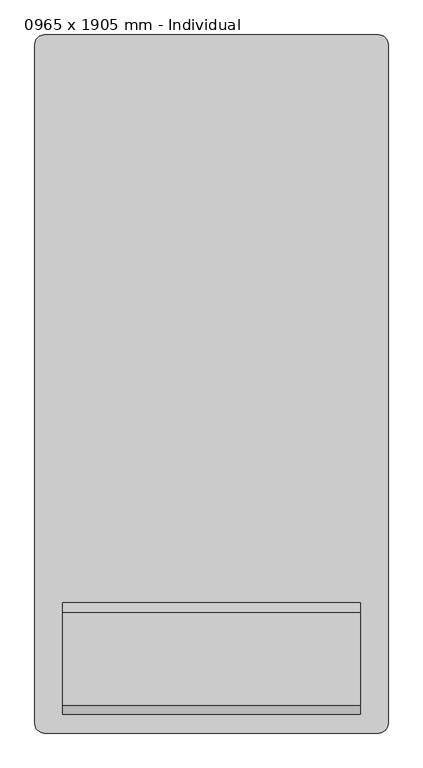
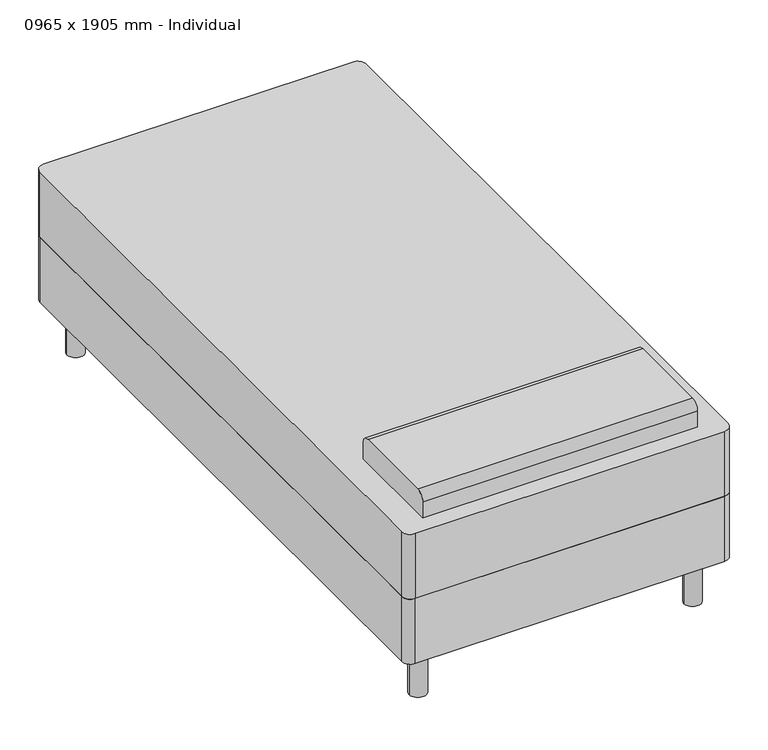
"""IFC4 building model written with IfcOpenShell, lengths in millimetres: furniture geometry, Cama-Estándar : 0965 x 1905 mm - Individual."""

from ifc_helpers import new_model, si_unit, point, frame, frame_2d, origin, origin_with_axes, place, context, project, spatial, polyline, circle_curve, trimmed, segment, composite_curve, outline, extrude, source, transform, mapped, element, save


def furniture_0965_x_1905_mm_individual_fedef34a(model_context):
    return source(origin(), model_context, "Body", "SweptSolid", [
        extrude(outline(composite_curve([segment(trimmed(circle_curve(frame_2d((-185.6114754, 972.695082)), 25.4), [point((-211.0114754, 972.695082))], [point((-185.6114754, 998.095082))], False, "CARTESIAN"), True, "CONTINUOUS"), segment(polyline([(-185.6114754, 998.095082), (728.5885246, 998.095082)]), True, "CONTINUOUS"), segment(trimmed(circle_curve(frame_2d((728.5885246, 972.695082)), 25.4), [point((728.5885246, 998.095082))], [point((753.9885246, 972.695082))], False, "CARTESIAN"), True, "CONTINUOUS"), segment(polyline([(753.9885246, 972.695082), (753.9885246, -881.504918)]), True, "CONTINUOUS"), segment(trimmed(circle_curve(frame_2d((728.5885246, -881.504918)), 25.4), [point((753.9885246, -881.504918))], [point((728.5885246, -906.904918))], False, "CARTESIAN"), True, "CONTINUOUS"), segment(polyline([(728.5885246, -906.904918), (-185.6114754, -906.904918)]), True, "CONTINUOUS"), segment(trimmed(circle_curve(frame_2d((-185.6114754, -881.504918)), 25.4), [point((-185.6114754, -906.904918))], [point((-211.0114754, -881.504918))], False, "CARTESIAN"), True, "CONTINUOUS"), segment(polyline([(-211.0114754, -881.504918), (-211.0114754, 972.695082)]), True, "CONTINUOUS")], self_intersect=False)), frame((0.0, 0.0, 152.4), z_axis=(0.0, 0.0, 1.0), x_axis=(1.0, 0.0, 0.0)), (0.0, 0.0, 1.0), 203.2),
        extrude(outline(composite_curve([segment(polyline([(-551.304918, 558.8), (-856.104918, 558.8), (-856.104918, 609.6)]), True, "CONTINUOUS"), segment(trimmed(circle_curve(frame_2d((-830.704918, 609.6)), 25.4), [point((-856.104918, 609.6))], [point((-830.704918, 635.0))], False, "CARTESIAN"), True, "CONTINUOUS"), segment(polyline([(-830.704918, 635.0), (-576.704918, 635.0)]), True, "CONTINUOUS"), segment(trimmed(circle_curve(frame_2d((-576.704918, 609.6)), 25.4), [point((-576.704918, 635.0))], [point((-551.304918, 609.6))], False, "CARTESIAN"), True, "CONTINUOUS"), segment(polyline([(-551.304918, 609.6), (-551.304918, 558.8)]), True, "CONTINUOUS")], self_intersect=False)), frame((-134.8114754, 0.0, 0.0), z_axis=(1.0, 0.0, 0.0), x_axis=(0.0, 1.0, 0.0)), (0.0, 0.0, 1.0), 812.6),
        extrude(outline(composite_curve([segment(trimmed(circle_curve(frame_2d((-134.8114754, -830.704918)), 25.4), [point((-160.2114754, -830.704918))], [point((-109.4114754, -830.704918))], False, "CARTESIAN"), True, "CONTINUOUS"), segment(trimmed(circle_curve(frame_2d((-134.8114754, -830.704918)), 25.4), [point((-109.4114754, -830.704918))], [point((-160.2114754, -830.704918))], False, "CARTESIAN"), True, "CONTINUOUS")], self_intersect=False)), origin_with_axes(), (0.0, 0.0, 1.0), 152.4),
        extrude(outline(composite_curve([segment(trimmed(circle_curve(frame_2d((677.7885246, -830.704918)), 25.4), [point((652.3885246, -830.704918))], [point((703.1885246, -830.704918))], False, "CARTESIAN"), True, "CONTINUOUS"), segment(trimmed(circle_curve(frame_2d((677.7885246, -830.704918)), 25.4), [point((703.1885246, -830.704918))], [point((652.3885246, -830.704918))], False, "CARTESIAN"), True, "CONTINUOUS")], self_intersect=False)), origin_with_axes(), (0.0, 0.0, 1.0), 152.4),
        extrude(outline(composite_curve([segment(trimmed(circle_curve(frame_2d((677.7885246, 921.895082)), 25.4), [point((652.3885246, 921.895082))], [point((703.1885246, 921.895082))], False, "CARTESIAN"), True, "CONTINUOUS"), segment(trimmed(circle_curve(frame_2d((677.7885246, 921.895082)), 25.4), [point((703.1885246, 921.895082))], [point((652.3885246, 921.895082))], False, "CARTESIAN"), True, "CONTINUOUS")], self_intersect=False)), origin_with_axes(), (0.0, 0.0, 1.0), 152.4),
        extrude(outline(composite_curve([segment(trimmed(circle_curve(frame_2d((-134.8114754, 921.895082)), 25.4), [point((-160.2114754, 921.895082))], [point((-109.4114754, 921.895082))], False, "CARTESIAN"), True, "CONTINUOUS"), segment(trimmed(circle_curve(frame_2d((-134.8114754, 921.895082)), 25.4), [point((-109.4114754, 921.895082))], [point((-160.2114754, 921.895082))], False, "CARTESIAN"), True, "CONTINUOUS")], self_intersect=False)), origin_with_axes(), (0.0, 0.0, 1.0), 152.4),
        extrude(outline(composite_curve([segment(trimmed(circle_curve(frame_2d((-185.6114754, -881.504918)), 25.4), [point((-185.6114754, -906.904918))], [point((-211.0114754, -881.504918))], False, "CARTESIAN"), True, "CONTINUOUS"), segment(polyline([(-211.0114754, -881.504918), (-211.0114754, 972.695082)]), True, "CONTINUOUS"), segment(trimmed(circle_curve(frame_2d((-185.6114754, 972.695082)), 25.4), [point((-211.0114754, 972.695082))], [point((-185.6114754, 998.095082))], False, "CARTESIAN"), True, "CONTINUOUS"), segment(polyline([(-185.6114754, 998.095082), (728.5885246, 998.095082)]), True, "CONTINUOUS"), segment(trimmed(circle_curve(frame_2d((728.5885246, 972.695082)), 25.4), [point((728.5885246, 998.095082))], [point((753.9885246, 972.695082))], False, "CARTESIAN"), True, "CONTINUOUS"), segment(polyline([(753.9885246, 972.695082), (753.9885246, -881.504918)]), True, "CONTINUOUS"), segment(trimmed(circle_curve(frame_2d((728.5885246, -881.504918)), 25.4), [point((753.9885246, -881.504918))], [point((728.5885246, -906.904918))], False, "CARTESIAN"), True, "CONTINUOUS"), segment(polyline([(728.5885246, -906.904918), (-185.6114754, -906.904918)]), True, "CONTINUOUS")], self_intersect=False)), frame((0.0, 0.0, 355.6), z_axis=(0.0, 0.0, 1.0), x_axis=(1.0, 0.0, 0.0)), (0.0, 0.0, 1.0), 203.2),
    ])


if __name__ == "__main__":
    model = new_model("IFC4")
    model_context = context("Model", 3, world=origin())
    ifc_project = project(units=[si_unit("LENGTHUNIT", "METRE", prefix="MILLI")], contexts=[model_context])
    site = spatial("IfcSite", under=ifc_project)
    building = spatial("IfcBuilding", under=site)
    placement = place(None, origin())
    furniture_0965_x_1905_mm_individual_shape = furniture_0965_x_1905_mm_individual_fedef34a(model_context)
    element("IfcFurniture", 1, ObjectType="Cama-Estándar : 0965 x 1905 mm - Individual", at=placement, inside=building, context=model_context, shape_type="MappedRepresentation", body=[
        mapped(furniture_0965_x_1905_mm_individual_shape, transform((0.0, 0.0, 0.0), x_axis=(1.0, 0.0, 0.0), y_axis=(0.0, 1.0, 0.0), z_axis=(0.0, 0.0, 1.0))),
    ])
    save(model, "model.ifc")

# Revit data of these elements
# Type "Cama-Estándar : 0965 x 1905 mm - Individual"
#   Longitud = 1.905 m
#   Anchura = 0.965 m
#   Máscara [instance default] = yes
#   Material de soporte = Metal - Cromo
#   Material de colchón = Textil - Blanco
#   Default Elevation = 0
# Element 1 (IfcFurniture, "Cama-Estándar : 0965 x 1905 mm - Individual")
#   Materials on its faces: "Metal - Cromo", "Textil - Blanco"
# Materials
#   "Metal - Cromo": class "Metal", colour RGB 17 17 17, transparency 0
#   "Textil - Blanco": class "Tela", colour RGB 247 247 239, transparency 0
